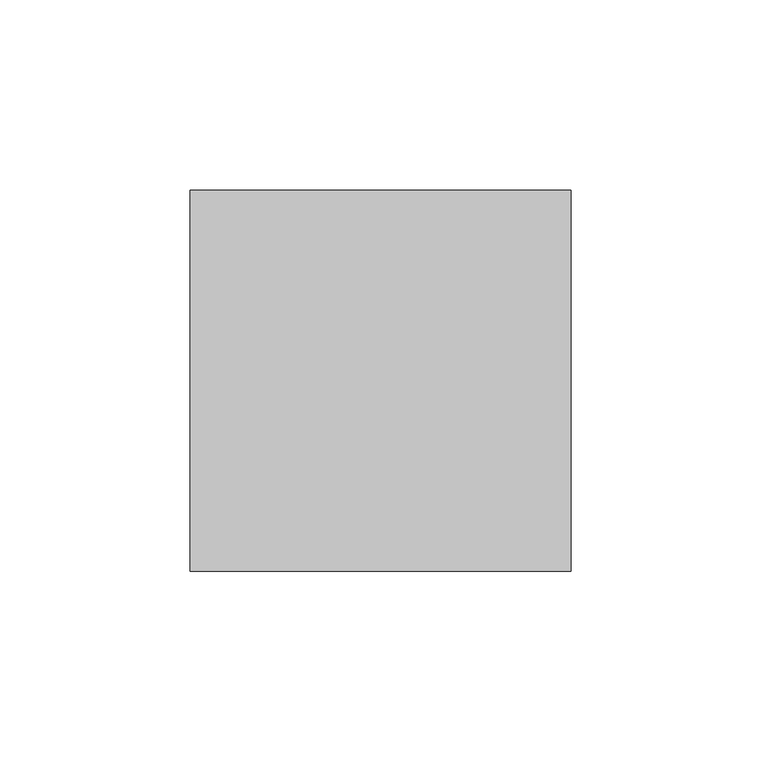
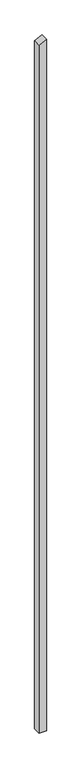
"""IFC4 building model written with IfcOpenShell, lengths in millimetres: column geometry, Holzstütze 159606 : Holzstütze 159606."""

from ifc_helpers import new_model, si_unit, frame, origin, place, context, project, spatial, polyline, outline, extrude, source, transform, mapped, element, save


def column_6093a7db(model_context):
    return source(origin(), model_context, "Body", "SweptSolid", [
        extrude(outline(polyline([(-500.0, 163237.7593015), (-500.0, 163337.7593015), (9423.2455407, 163337.7593015), (9372.2929958, 163237.7593015), (-500.0, 163237.7593015)])), frame((0.0, 26981.9343946, 0.0), z_axis=(0.0, 1.0, 0.0), x_axis=(0.0, 0.0, 1.0)), (0.0, 0.0, 1.0), 100.0),
    ])


if __name__ == "__main__":
    model = new_model("IFC4")
    model_context = context("Model", 3, world=origin())
    ifc_project = project(units=[si_unit("LENGTHUNIT", "METRE", prefix="MILLI")], contexts=[model_context])
    site = spatial("IfcSite", under=ifc_project)
    building = spatial("IfcBuilding", under=site)
    placement = place(None, origin())
    column_shape = column_6093a7db(model_context)
    element("IfcColumn", 1, ObjectType="Holzstütze 159606 : Holzstütze 159606", at=placement, inside=building, context=model_context, shape_type="MappedRepresentation", body=[
        mapped(column_shape, transform((0.0, 0.0, 0.0), x_axis=(1.0, 0.0, 0.0), y_axis=(0.0, 1.0, 0.0), z_axis=(0.0, 0.0, 1.0))),
    ])
    save(model, "model.ifc")

# Revit data of these elements
# Type "Holzstütze 159606 : Holzstütze 159606"
#   Abrechnungsart = "m"
#   Allright_Bauteil_ID = "0152St 0000143460"
#   Bezeichnung = "Holzstütze"
#   Codetext = "ST-HOLZ\\"
#   Gewerk = "Zimmer- und Holzbauarbeiten"
#   Material = "Holz"
#   Objektname = "Stütze"
#   NameOverride = "Holzstütze"
#   Reference = "Holzstütze"
#   Status = "NEW"
#   ThermalTransmittance = 0.0000 BTU/(h·ft²·°F)
#   Roll = 0.00°
#   Slope = 0.00°
#   2D Interaktion = yes
#   IsExternal = yes
#   LoadBearing = yes
# Element 1 (IfcColumn, "Holzstütze 159606 : Holzstütze 159606")
#   Materials on its faces: "holzschalung"
# Materials
#   "holzschalung": class "Unassigned", colour RGB 128 128 128, transparency 0
